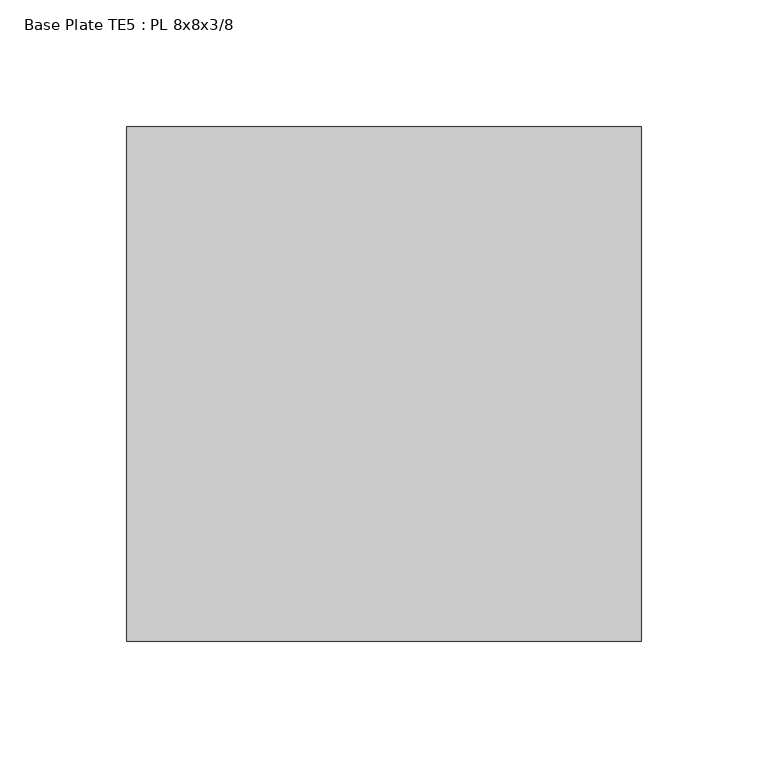
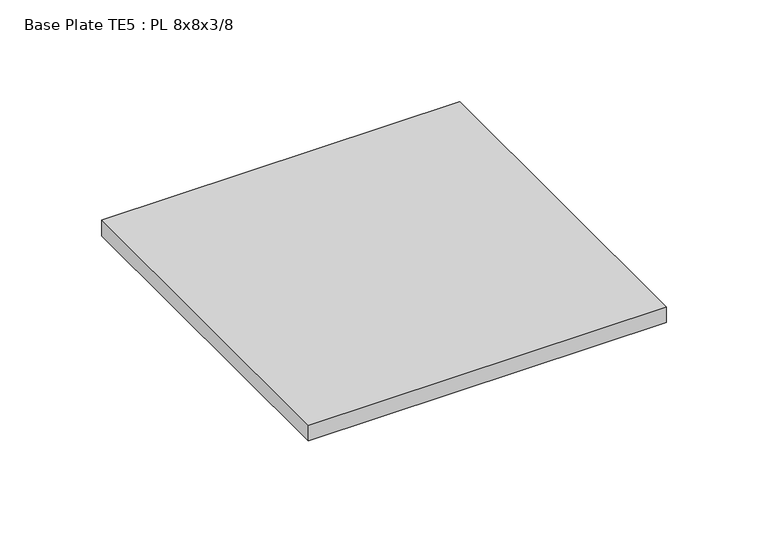
"""IFC4 building model written with IfcOpenShell, lengths in millimetres: proxy geometry, Base Plate TE5 : PL 8x8x3/8."""

import ifcopenshell
import ifcopenshell.guid

model = None  # the IFC model being written
_history = None  # IfcOwnerHistory: only IFC2X3 demands one
_inside = {}  # id of a spatial element -> (the spatial element, [elements in it])
_under = {}  # id of a project, library or spatial element -> (it, [spatial elements below it])
_declared = {}  # id of a project -> (the project, [libraries it declares])
_typed = {}  # id of a type object -> (the type object, [elements of that type])
_made_of = {}  # id of a material, layer set ... -> (it, [elements and type objects made of it])


def new_model(schema):
    """Start an empty IFC model of exactly this schema.

    Asked for "IFC4X3", IfcOpenShell would pick the latest addendum, in which some entities
    have other attributes; the version numbers below select the first issue.
    IFC2X3 requires an IfcOwnerHistory on every rooted entity: one is made here for all.
    """
    global model, _history
    if schema == "IFC4X3":
        model = ifcopenshell.file(schema_version=(4, 3, 0, 0))
    else:
        model = ifcopenshell.file(schema=schema)
    _inside.clear()
    _under.clear()
    _declared.clear()
    _typed.clear()
    _made_of.clear()
    _history = None
    if model.schema == "IFC2X3":
        org = make("IfcOrganization", Name="unknown")
        user = make(
            "IfcPersonAndOrganization",
            ThePerson=make("IfcPerson", FamilyName="unknown"),
            TheOrganization=org,
        )
        app = make(
            "IfcApplication",
            ApplicationDeveloper=org,
            Version="unknown",
            ApplicationFullName="unknown",
            ApplicationIdentifier="unknown",
        )
        _history = make(
            "IfcOwnerHistory",
            OwningUser=user,
            OwningApplication=app,
            ChangeAction="ADDED",
            CreationDate=0,
        )
    return model


def make(cls, **values):
    """One entity of the class cls with the attributes given. An attribute that is None is left unset."""
    return model.create_entity(
        cls, **{name: value for name, value in values.items() if value is not None}
    )


def rooted(cls, **values):
    """An entity with a GlobalId (a new one), such as an element, a storey or a relation."""
    return make(cls, GlobalId=ifcopenshell.guid.new(), OwnerHistory=_history, **values)


def si_unit(unit_type, name, prefix=None):
    """IfcSIUnit, for example si_unit("LENGTHUNIT", "METRE", prefix="MILLI")."""
    return make("IfcSIUnit", UnitType=unit_type, Prefix=prefix, Name=name)


def assignment(units):
    """IfcUnitAssignment: the units of a project."""
    return None if units is None else make("IfcUnitAssignment", Units=units)


def point(xyz):
    """IfcCartesianPoint."""
    return None if xyz is None else make("IfcCartesianPoint", Coordinates=xyz)


def direction(xyz):
    """IfcDirection."""
    return None if xyz is None else make("IfcDirection", DirectionRatios=xyz)


def frame(location, z_axis=None, x_axis=None):
    """IfcAxis2Placement3D, a coordinate frame: its origin and axes. An axis left out is left unset."""
    return make(
        "IfcAxis2Placement3D",
        Location=point(location),
        Axis=direction(z_axis),
        RefDirection=direction(x_axis),
    )


def origin():
    """The frame at (0, 0, 0) with its axes left unset."""
    return frame((0.0, 0.0, 0.0))


def place(relative_to, where):
    """IfcLocalPlacement: puts the frame where relative to a parent placement (None: the world)."""
    return make(
        "IfcLocalPlacement", PlacementRelTo=relative_to, RelativePlacement=where
    )


def context(
    kind, dimensions, precision=None, world=None, true_north=None, identifier=None
):
    """IfcGeometricRepresentationContext, for example the 3D "Model" context."""
    return make(
        "IfcGeometricRepresentationContext",
        ContextIdentifier=identifier,
        ContextType=kind,
        CoordinateSpaceDimension=dimensions,
        Precision=precision,
        WorldCoordinateSystem=world,
        TrueNorth=true_north,
    )


def project(units=None, contexts=None):
    """IfcProject with its units and contexts."""
    return rooted(
        "IfcProject",
        Name="project",
        RepresentationContexts=contexts,
        UnitsInContext=assignment(units),
    )


def spatial(cls, under=None, at=None, **own):
    """A site, building, storey or space (cls), placed at a placement, below another one or the project."""
    s = rooted(cls, ObjectPlacement=at, **own)
    if under is not None:
        _under.setdefault(under.id(), (under, []))[1].append(s)
    return s


def polyline(points):
    """IfcPolyline through the points."""
    return make("IfcPolyline", Points=[point(p) for p in points])


def outline(outer, holes=None, kind="AREA"):
    """IfcArbitraryClosedProfileDef: a profile drawn as a closed curve; with holes, ...WithVoids."""
    if holes is None:
        return make("IfcArbitraryClosedProfileDef", ProfileType=kind, OuterCurve=outer)
    return make(
        "IfcArbitraryProfileDefWithVoids",
        ProfileType=kind,
        OuterCurve=outer,
        InnerCurves=holes,
    )


def extrude(swept, where, along, depth):
    """IfcExtrudedAreaSolid: the profile swept, set in the frame where, extruded along a direction by depth."""
    return make(
        "IfcExtrudedAreaSolid",
        SweptArea=swept,
        Position=where,
        ExtrudedDirection=direction(along),
        Depth=depth,
    )


def shape(context_of_items, identifier, shape_type, items):
    """IfcShapeRepresentation: the items that make up one representation, for example the "Body"."""
    return make(
        "IfcShapeRepresentation",
        ContextOfItems=context_of_items,
        RepresentationIdentifier=identifier,
        RepresentationType=shape_type,
        Items=items,
    )


def source(mapping_origin, context_of_items, identifier, shape_type, items):
    """IfcRepresentationMap: a shape defined once, which mapped items show again and again."""
    return make(
        "IfcRepresentationMap",
        MappingOrigin=mapping_origin,
        MappedRepresentation=shape(context_of_items, identifier, shape_type, items),
    )


def transform(
    local_origin,
    x_axis=None,
    y_axis=None,
    z_axis=None,
    scale=None,
    scale2=None,
    scale3=None,
    uniform=True,
):
    """IfcCartesianTransformationOperator3D, or its non-uniform kind. x_axis, y_axis, z_axis: its Axis1, 2, 3."""
    if uniform:
        return make(
            "IfcCartesianTransformationOperator3D",
            Axis1=direction(x_axis),
            Axis2=direction(y_axis),
            LocalOrigin=point(local_origin),
            Scale=scale,
            Axis3=direction(z_axis),
        )
    return make(
        "IfcCartesianTransformationOperator3DnonUniform",
        Axis1=direction(x_axis),
        Axis2=direction(y_axis),
        LocalOrigin=point(local_origin),
        Scale=scale,
        Axis3=direction(z_axis),
        Scale2=scale2,
        Scale3=scale3,
    )


def mapped(mapping_source, mapping_target):
    """IfcMappedItem: shows the shape of a source again, moved by a transform."""
    return make(
        "IfcMappedItem", MappingSource=mapping_source, MappingTarget=mapping_target
    )


def made_of(thing, what):
    """Note that an element or type object is made of a material, layer set ...; save() writes the relation."""
    if what is not None:
        _made_of.setdefault(what.id(), (what, []))[1].append(thing)
    return thing


def element(
    cls,
    number,
    at=None,
    inside=None,
    cuts=None,
    type_object=None,
    material=None,
    context=None,
    identifier="Body",
    shape_type=None,
    held_by="IfcProductDefinitionShape",
    body=None,
    shapes=None,
    **own,
):
    """One element of the class cls, such as IfcWall. Its Tag is "e" and its number.

    at: its placement. inside: the storey or other place that contains it. cuts: it is an
    opening in that element (IfcRelVoidsElement). A single representation is given by context,
    identifier, shape_type and body (its items); several are given by shapes. held_by: the class
    of the entity that holds the representations. save() writes the other relations.
    """
    e = rooted(cls, Tag="e%d" % number, ObjectPlacement=at, **own)
    if body is not None:
        shapes = [shape(context, identifier, shape_type, body)]
    if shapes is not None:
        e.Representation = make(held_by, Representations=shapes)
    if inside is not None:
        _inside.setdefault(inside.id(), (inside, []))[1].append(e)
    if cuts is not None:
        rooted(
            "IfcRelVoidsElement", RelatingBuildingElement=cuts, RelatedOpeningElement=e
        )
    if type_object is not None:
        _typed.setdefault(type_object.id(), (type_object, []))[1].append(e)
    return made_of(e, material)


def aggregate(whole, parts):
    """IfcRelAggregates: a whole, such as a stair, and the parts it consists of."""
    return rooted("IfcRelAggregates", RelatingObject=whole, RelatedObjects=parts)


def save(model, path):
    """Write the relations noted so far, then the file.

    IfcRelAggregates (storeys below a building ...), IfcRelContainedInSpatialStructure (elements
    in a storey), IfcRelDefinesByType, IfcRelAssociatesMaterial and IfcRelDeclares: one each for
    every whole, place, type object, material and project.
    """
    for whole, parts in _under.values():
        aggregate(whole, parts)
    for where, things in _inside.values():
        rooted(
            "IfcRelContainedInSpatialStructure",
            RelatedElements=things,
            RelatingStructure=where,
        )
    for kind, things in _typed.values():
        rooted("IfcRelDefinesByType", RelatedObjects=things, RelatingType=kind)
    for what, things in _made_of.values():
        rooted("IfcRelAssociatesMaterial", RelatedObjects=things, RelatingMaterial=what)
    for by, libraries in _declared.values():
        rooted("IfcRelDeclares", RelatingContext=by, RelatedDefinitions=libraries)
    model.write(path)


def base_plate_te5_pl_8x8x3_8_4141263b(model_context):
    return source(origin(), model_context, "Body", "SweptSolid", [
        extrude(outline(polyline([(587365.8770246, -536468.3913841), (587365.8770246, -536265.1913841), (587569.0770246, -536265.1913841), (587569.0770246, -536468.3913841), (587365.8770246, -536468.3913841)])), frame((0.0, 0.0, 19.05), z_axis=(0.0, 0.0, 1.0), x_axis=(1.0, 0.0, 0.0)), (0.0, 0.0, 1.0), 9.525),
    ])


if __name__ == "__main__":
    model = new_model("IFC4")
    model_context = context("Model", 3, world=origin())
    ifc_project = project(units=[si_unit("LENGTHUNIT", "METRE", prefix="MILLI")], contexts=[model_context])
    site = spatial("IfcSite", under=ifc_project)
    building = spatial("IfcBuilding", under=site)
    placement = place(None, origin())
    base_plate_te5_pl_8x8x3_8_shape = base_plate_te5_pl_8x8x3_8_4141263b(model_context)
    element("IfcBuildingElementProxy", 1, Name="Base Plate TE5 : PL 8x8x3/8", ObjectType="Base Plate TE5 : PL 8x8x3/8", at=placement, inside=building, context=model_context, shape_type="MappedRepresentation", body=[
        mapped(base_plate_te5_pl_8x8x3_8_shape, transform((0.0, 0.0, 0.0), x_axis=(1.0, 0.0, 0.0), y_axis=(0.0, 1.0, 0.0), z_axis=(0.0, 0.0, 1.0))),
    ])
    save(model, "model.ifc")

# Revit data of these elements
# Element 1 (IfcBuildingElementProxy, "Base Plate TE5 : PL 8x8x3/8")
#   Materials on its faces: "GALV. STL BASE PLATE"
# Materials
#   "GALV. STL BASE PLATE": class "Generic", colour RGB 211 211 207, transparency 0, Cost = 0
